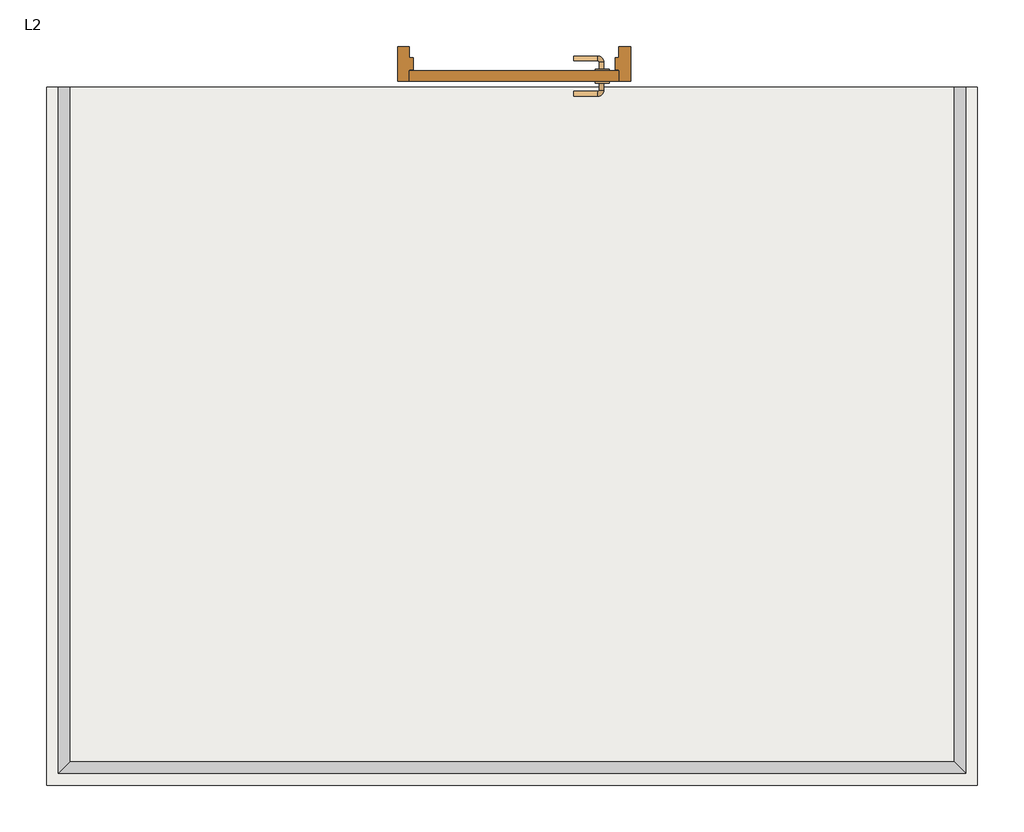
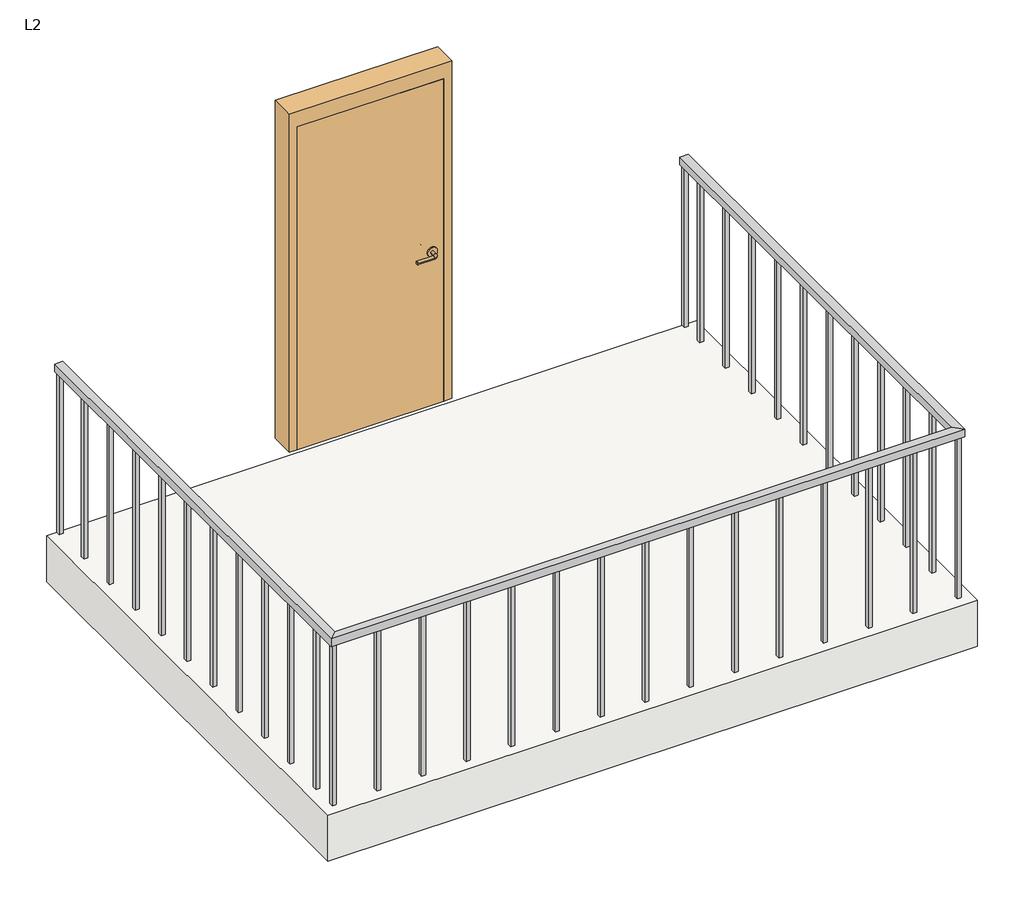
# One storey: 1 door, 1 railing, 1 slab.
"""IFC4 building model written with IfcOpenShell, lengths in millimetres."""

import ifcopenshell
import ifcopenshell.guid

model = None  # the IFC model being written
_history = None  # IfcOwnerHistory: only IFC2X3 demands one
_inside = {}  # id of a spatial element -> (the spatial element, [elements in it])
_under = {}  # id of a project, library or spatial element -> (it, [spatial elements below it])
_declared = {}  # id of a project -> (the project, [libraries it declares])
_typed = {}  # id of a type object -> (the type object, [elements of that type])
_made_of = {}  # id of a material, layer set ... -> (it, [elements and type objects made of it])


def new_model(schema):
    """Start an empty IFC model of exactly this schema.

    Asked for "IFC4X3", IfcOpenShell would pick the latest addendum, in which some entities
    have other attributes; the version numbers below select the first issue.
    IFC2X3 requires an IfcOwnerHistory on every rooted entity: one is made here for all.
    """
    global model, _history
    if schema == "IFC4X3":
        model = ifcopenshell.file(schema_version=(4, 3, 0, 0))
    else:
        model = ifcopenshell.file(schema=schema)
    _inside.clear()
    _under.clear()
    _declared.clear()
    _typed.clear()
    _made_of.clear()
    _history = None
    if model.schema == "IFC2X3":
        org = make("IfcOrganization", Name="unknown")
        user = make(
            "IfcPersonAndOrganization",
            ThePerson=make("IfcPerson", FamilyName="unknown"),
            TheOrganization=org,
        )
        app = make(
            "IfcApplication",
            ApplicationDeveloper=org,
            Version="unknown",
            ApplicationFullName="unknown",
            ApplicationIdentifier="unknown",
        )
        _history = make(
            "IfcOwnerHistory",
            OwningUser=user,
            OwningApplication=app,
            ChangeAction="ADDED",
            CreationDate=0,
        )
    return model


def make(cls, **values):
    """One entity of the class cls with the attributes given. An attribute that is None is left unset."""
    return model.create_entity(
        cls, **{name: value for name, value in values.items() if value is not None}
    )


def rooted(cls, **values):
    """An entity with a GlobalId (a new one), such as an element, a storey or a relation."""
    return make(cls, GlobalId=ifcopenshell.guid.new(), OwnerHistory=_history, **values)


def si_unit(unit_type, name, prefix=None):
    """IfcSIUnit, for example si_unit("LENGTHUNIT", "METRE", prefix="MILLI")."""
    return make("IfcSIUnit", UnitType=unit_type, Prefix=prefix, Name=name)


def assignment(units):
    """IfcUnitAssignment: the units of a project."""
    return None if units is None else make("IfcUnitAssignment", Units=units)


def point(xyz):
    """IfcCartesianPoint."""
    return None if xyz is None else make("IfcCartesianPoint", Coordinates=xyz)


def direction(xyz):
    """IfcDirection."""
    return None if xyz is None else make("IfcDirection", DirectionRatios=xyz)


def frame(location, z_axis=None, x_axis=None):
    """IfcAxis2Placement3D, a coordinate frame: its origin and axes. An axis left out is left unset."""
    return make(
        "IfcAxis2Placement3D",
        Location=point(location),
        Axis=direction(z_axis),
        RefDirection=direction(x_axis),
    )


def frame_2d(location, x_axis=None):
    """IfcAxis2Placement2D, a coordinate frame in the plane: its origin and x axis."""
    return make(
        "IfcAxis2Placement2D", Location=point(location), RefDirection=direction(x_axis)
    )


def origin():
    """The frame at (0, 0, 0) with its axes left unset."""
    return frame((0.0, 0.0, 0.0))


def origin_with_axes():
    """The frame at (0, 0, 0) with the z axis (0, 0, 1) and the x axis (1, 0, 0) written out."""
    return frame((0.0, 0.0, 0.0), z_axis=(0.0, 0.0, 1.0), x_axis=(1.0, 0.0, 0.0))


def place(relative_to, where):
    """IfcLocalPlacement: puts the frame where relative to a parent placement (None: the world)."""
    return make(
        "IfcLocalPlacement", PlacementRelTo=relative_to, RelativePlacement=where
    )


def context(
    kind, dimensions, precision=None, world=None, true_north=None, identifier=None
):
    """IfcGeometricRepresentationContext, for example the 3D "Model" context."""
    return make(
        "IfcGeometricRepresentationContext",
        ContextIdentifier=identifier,
        ContextType=kind,
        CoordinateSpaceDimension=dimensions,
        Precision=precision,
        WorldCoordinateSystem=world,
        TrueNorth=true_north,
    )


def project(units=None, contexts=None):
    """IfcProject with its units and contexts."""
    return rooted(
        "IfcProject",
        Name="project",
        RepresentationContexts=contexts,
        UnitsInContext=assignment(units),
    )


def spatial(cls, under=None, at=None, **own):
    """A site, building, storey or space (cls), placed at a placement, below another one or the project."""
    s = rooted(cls, ObjectPlacement=at, **own)
    if under is not None:
        _under.setdefault(under.id(), (under, []))[1].append(s)
    return s


def polyline(points):
    """IfcPolyline through the points."""
    return make("IfcPolyline", Points=[point(p) for p in points])


def circle_curve(where, radius):
    """IfcCircle in the frame where."""
    return make("IfcCircle", Position=where, Radius=radius)


def ellipse_curve(where, semi_axis1, semi_axis2):
    """IfcEllipse in the frame where."""
    return make(
        "IfcEllipse", Position=where, SemiAxis1=semi_axis1, SemiAxis2=semi_axis2
    )


def trimmed(basis, trim1, trim2, sense, master):
    """IfcTrimmedCurve: the piece of a basis curve between two trims."""
    return make(
        "IfcTrimmedCurve",
        BasisCurve=basis,
        Trim1=trim1,
        Trim2=trim2,
        SenseAgreement=sense,
        MasterRepresentation=master,
    )


def segment(curve, same_sense, transition):
    """IfcCompositeCurveSegment."""
    return make(
        "IfcCompositeCurveSegment",
        Transition=transition,
        SameSense=same_sense,
        ParentCurve=curve,
    )


def composite_curve(segments, self_intersect=None):
    """IfcCompositeCurve: segments joined end to end."""
    return make("IfcCompositeCurve", Segments=segments, SelfIntersect=self_intersect)


def outline(outer, holes=None, kind="AREA"):
    """IfcArbitraryClosedProfileDef: a profile drawn as a closed curve; with holes, ...WithVoids."""
    if holes is None:
        return make("IfcArbitraryClosedProfileDef", ProfileType=kind, OuterCurve=outer)
    return make(
        "IfcArbitraryProfileDefWithVoids",
        ProfileType=kind,
        OuterCurve=outer,
        InnerCurves=holes,
    )


def extrude(swept, where, along, depth):
    """IfcExtrudedAreaSolid: the profile swept, set in the frame where, extruded along a direction by depth."""
    return make(
        "IfcExtrudedAreaSolid",
        SweptArea=swept,
        Position=where,
        ExtrudedDirection=direction(along),
        Depth=depth,
    )


def faces_of(points, faces, orient=None, outer=None):
    """IfcFace entities. A face is a list of loops; a loop is a list of indices into points, from 0.

    orient and outer hold one flag for each loop. By default every Orientation is true, the
    first loop of a face is its IfcFaceOuterBound and the others are IfcFaceBound.
    """
    made = []
    for i, loops in enumerate(faces):
        bounds = []
        for j, loop in enumerate(loops):
            is_outer = j == 0 if outer is None else outer[i][j]
            bounds.append(
                make(
                    "IfcFaceOuterBound" if is_outer else "IfcFaceBound",
                    Bound=make("IfcPolyLoop", Polygon=[points[k] for k in loop]),
                    Orientation=True if orient is None else orient[i][j],
                )
            )
        made.append(make("IfcFace", Bounds=bounds))
    return made


def faceted_brep(points, faces, orient=None, outer=None, voids=None):
    """IfcFacetedBrep: a solid bounded by flat faces; with voids (closed shells), ...WithVoids."""
    shared = [point(p) for p in points]
    hull = make("IfcClosedShell", CfsFaces=faces_of(shared, faces, orient, outer))
    if voids is None:
        return make("IfcFacetedBrep", Outer=hull)
    return make(
        "IfcFacetedBrepWithVoids",
        Outer=hull,
        Voids=[
            make(cls, CfsFaces=faces_of(shared, fs, o, b)) for cls, fs, o, b in voids
        ],
    )


def shape(context_of_items, identifier, shape_type, items):
    """IfcShapeRepresentation: the items that make up one representation, for example the "Body"."""
    return make(
        "IfcShapeRepresentation",
        ContextOfItems=context_of_items,
        RepresentationIdentifier=identifier,
        RepresentationType=shape_type,
        Items=items,
    )


def source(mapping_origin, context_of_items, identifier, shape_type, items):
    """IfcRepresentationMap: a shape defined once, which mapped items show again and again."""
    return make(
        "IfcRepresentationMap",
        MappingOrigin=mapping_origin,
        MappedRepresentation=shape(context_of_items, identifier, shape_type, items),
    )


def transform(
    local_origin,
    x_axis=None,
    y_axis=None,
    z_axis=None,
    scale=None,
    scale2=None,
    scale3=None,
    uniform=True,
):
    """IfcCartesianTransformationOperator3D, or its non-uniform kind. x_axis, y_axis, z_axis: its Axis1, 2, 3."""
    if uniform:
        return make(
            "IfcCartesianTransformationOperator3D",
            Axis1=direction(x_axis),
            Axis2=direction(y_axis),
            LocalOrigin=point(local_origin),
            Scale=scale,
            Axis3=direction(z_axis),
        )
    return make(
        "IfcCartesianTransformationOperator3DnonUniform",
        Axis1=direction(x_axis),
        Axis2=direction(y_axis),
        LocalOrigin=point(local_origin),
        Scale=scale,
        Axis3=direction(z_axis),
        Scale2=scale2,
        Scale3=scale3,
    )


def mapped(mapping_source, mapping_target):
    """IfcMappedItem: shows the shape of a source again, moved by a transform."""
    return make(
        "IfcMappedItem", MappingSource=mapping_source, MappingTarget=mapping_target
    )


def made_of(thing, what):
    """Note that an element or type object is made of a material, layer set ...; save() writes the relation."""
    if what is not None:
        _made_of.setdefault(what.id(), (what, []))[1].append(thing)
    return thing


def element(
    cls,
    number,
    at=None,
    inside=None,
    cuts=None,
    type_object=None,
    material=None,
    context=None,
    identifier="Body",
    shape_type=None,
    held_by="IfcProductDefinitionShape",
    body=None,
    shapes=None,
    **own,
):
    """One element of the class cls, such as IfcWall. Its Tag is "e" and its number.

    at: its placement. inside: the storey or other place that contains it. cuts: it is an
    opening in that element (IfcRelVoidsElement). A single representation is given by context,
    identifier, shape_type and body (its items); several are given by shapes. held_by: the class
    of the entity that holds the representations. save() writes the other relations.
    """
    e = rooted(cls, Tag="e%d" % number, ObjectPlacement=at, **own)
    if body is not None:
        shapes = [shape(context, identifier, shape_type, body)]
    if shapes is not None:
        e.Representation = make(held_by, Representations=shapes)
    if inside is not None:
        _inside.setdefault(inside.id(), (inside, []))[1].append(e)
    if cuts is not None:
        rooted(
            "IfcRelVoidsElement", RelatingBuildingElement=cuts, RelatedOpeningElement=e
        )
    if type_object is not None:
        _typed.setdefault(type_object.id(), (type_object, []))[1].append(e)
    return made_of(e, material)


def aggregate(whole, parts):
    """IfcRelAggregates: a whole, such as a stair, and the parts it consists of."""
    return rooted("IfcRelAggregates", RelatingObject=whole, RelatedObjects=parts)


def save(model, path):
    """Write the relations noted so far, then the file.

    IfcRelAggregates (storeys below a building ...), IfcRelContainedInSpatialStructure (elements
    in a storey), IfcRelDefinesByType, IfcRelAssociatesMaterial and IfcRelDeclares: one each for
    every whole, place, type object, material and project.
    """
    for whole, parts in _under.values():
        aggregate(whole, parts)
    for where, things in _inside.values():
        rooted(
            "IfcRelContainedInSpatialStructure",
            RelatedElements=things,
            RelatingStructure=where,
        )
    for kind, things in _typed.values():
        rooted("IfcRelDefinesByType", RelatedObjects=things, RelatingType=kind)
    for what, things in _made_of.values():
        rooted("IfcRelAssociatesMaterial", RelatedObjects=things, RelatingMaterial=what)
    for by, libraries in _declared.values():
        rooted("IfcRelDeclares", RelatingContext=by, RelatedDefinitions=libraries)
    model.write(path)


def plane_surface(at):
    """IfcPlane: the flat surface through the origin of the frame at, square to its z axis."""
    return make("IfcPlane", Position=at)


def cylinder_surface(at, radius):
    """IfcCylindricalSurface: all points at the distance radius from the z axis of the frame at."""
    return make("IfcCylindricalSurface", Position=at, Radius=radius)


def revolved_surface(curve, axis_point, axis_direction):
    """IfcSurfaceOfRevolution: the curve turned about the line through axis_point along axis_direction."""
    return make(
        "IfcSurfaceOfRevolution",
        SweptCurve=make("IfcArbitraryOpenProfileDef", ProfileType="CURVE", Curve=curve),
        AxisPosition=make("IfcAxis1Placement", Location=point(axis_point), Axis=direction(axis_direction)),
    )


def advanced_brep(points, edges, surfaces, faces):
    """IfcAdvancedBrep: a solid bounded by faces that lie on surfaces and meet in shared edges.

    An edge is (start, end): straight between two places in points (the first is 0);
    or (start, end, curve); or (start, end, curve, False) where it runs against its curve.
    A face is (place in surfaces, loops), or (place, loops, False) where it looks against
    its surface's normal. A loop lists edges by number (the first is 1), with a minus sign
    where the edge is run from its end to its start. The first loop is the outer one.
    """
    corners = [point(p) for p in points]
    vertices = [make("IfcVertexPoint", VertexGeometry=c) for c in corners]
    made = []
    for start, end, *more in edges:
        made.append(
            make(
                "IfcEdgeCurve",
                EdgeStart=vertices[start],
                EdgeEnd=vertices[end],
                EdgeGeometry=more[0] if more else make("IfcPolyline", Points=[corners[start], corners[end]]),
                SameSense=more[1] if len(more) > 1 else True,
            )
        )
    hull = []
    for where, loops, *sense in faces:
        bounds = []
        for j, loop in enumerate(loops):
            ring = [make("IfcOrientedEdge", EdgeElement=made[abs(k) - 1], Orientation=k > 0) for k in loop]
            bounds.append(
                make(
                    "IfcFaceOuterBound" if j == 0 else "IfcFaceBound",
                    Bound=make("IfcEdgeLoop", EdgeList=ring),
                    Orientation=True,
                )
            )
        hull.append(make("IfcAdvancedFace", Bounds=bounds, FaceSurface=surfaces[where], SameSense=sense[0] if sense else True))
    return make("IfcAdvancedBrep", Outer=make("IfcClosedShell", CfsFaces=hull))


def m_door_passage_single_flush_900_x_2100mm_f70d95c9(model_context):
    return source(origin(), model_context, "Body", "SolidModel", [
        advanced_brep(
        [(-384.990625, 3.35, 1000.0), (-364.990625, 3.35, 1000.0), (-364.990625, -26.65, 1000.0), (-384.990625, -26.65, 1000.0), (-359.990625, -31.65, 1000.0), (-359.990625, -51.65, 1000.0), (-254.990625, -51.65, 1000.0), (-254.990625, -31.65, 1000.0)],
        [
            (0, 1, circle_curve(frame((-374.990625, 3.35, 1000.0), z_axis=(0.0, 1.0, 0.0), x_axis=(1.0, 0.0, 0.0)), 10.0)),
            (1, 0, circle_curve(frame((-374.990625, 3.35, 1000.0), z_axis=(0.0, 1.0, 0.0), x_axis=(1.0, 0.0, 0.0)), 10.0)),
            (1, 2),
            (2, 3, circle_curve(frame((-374.990625, -26.65, 1000.0), z_axis=(0.0, 1.0, 0.0), x_axis=(1.0, 0.0, 0.0)), 10.0)),
            (3, 0),
            (3, 2, circle_curve(frame((-374.990625, -26.65, 1000.0), z_axis=(0.0, 1.0, 0.0), x_axis=(1.0, 0.0, 0.0)), 10.0)),
            (4, 5, circle_curve(frame((-359.990625, -41.65, 1000.0), z_axis=(-1.0, 0.0, 0.0), x_axis=(0.0, 1.0, 0.0)), 10.0)),
            (5, 3, circle_curve(frame((-359.990625, -26.65, 1000.0), z_axis=(0.0, 0.0, -1.0), x_axis=(-1.0, 0.0, 0.0)), 25.0)),
            (2, 4, circle_curve(frame((-359.990625, -26.65, 1000.0), z_axis=(0.0, 0.0, 1.0), x_axis=(-1.0, 0.0, 0.0)), 5.0)),
            (5, 4, circle_curve(frame((-359.990625, -41.65, 1000.0), z_axis=(-1.0, 0.0, 0.0), x_axis=(0.0, 1.0, 0.0)), 10.0)),
            (6, 7, circle_curve(frame((-254.990625, -41.65, 1000.0), z_axis=(1.0, 0.0, 0.0), x_axis=(0.0, 1.0, 0.0)), 10.0)),
            (7, 6, circle_curve(frame((-254.990625, -41.65, 1000.0), z_axis=(1.0, 0.0, 0.0), x_axis=(0.0, 1.0, 0.0)), 10.0)),
            (4, 7),
            (6, 5),
        ],
        [
            plane_surface(frame((-374.990625, 3.35, 1000.0), z_axis=(0.0, 1.0, 0.0), x_axis=(0.0, 0.0, 1.0))),
            cylinder_surface(frame((-374.990625, 3.35, 1000.0), z_axis=(0.0, 1.0, 0.0), x_axis=(1.0, 0.0, 0.0)), 10.0),
            revolved_surface(trimmed(ellipse_curve(frame((-374.990625, -26.65, 1000.0), z_axis=(0.0, -1.0, 0.0), x_axis=(1.0, 0.0, 0.0)), 10.0, 10.0), [point((-384.990625, -26.65, 1000.0))], [point((-364.990625, -26.65, 1000.0))], True, "CARTESIAN"), (-359.990625, -26.65, 1000.0), (0.0, 0.0, -1.0)),
            revolved_surface(trimmed(ellipse_curve(frame((-374.990625, -26.65, 1000.0), z_axis=(0.0, -1.0, 0.0), x_axis=(1.0, 0.0, 0.0)), 10.0, 10.0), [point((-364.990625, -26.65, 1000.0))], [point((-384.990625, -26.65, 1000.0))], True, "CARTESIAN"), (-359.990625, -26.65, 1000.0), (0.0, 0.0, -1.0)),
            plane_surface(frame((-254.990625, -41.65, 1000.0), z_axis=(1.0, 0.0, 0.0), x_axis=(0.0, 0.0, 1.0))),
            cylinder_surface(frame((-359.990625, -41.65, 1000.0), z_axis=(-1.0, 0.0, 0.0), x_axis=(0.0, 1.0, 0.0)), 10.0),
        ],
        [
            (0, [[1, 2]]),
            (1, [[3, 4, 5, -2]]),
            (1, [[-5, 6, -3, -1]]),
            (2, [[7, 8, -4, 9]]),
            (3, [[10, -9, -6, -8]]),
            (4, [[11, 12]]),
            (5, [[13, -11, 14, -7]]),
            (5, [[-14, -12, -13, -10]]),
        ],
    ),
        extrude(outline(composite_curve([segment(trimmed(circle_curve(frame_2d((1000.0, -377.490625)), 30.0), [point((1000.0, -407.490625))], [point((1000.0, -347.490625))], False, "CARTESIAN"), True, "CONTINUOUS"), segment(trimmed(circle_curve(frame_2d((1000.0, -377.490625)), 30.0), [point((1000.0, -347.490625))], [point((1000.0, -407.490625))], False, "CARTESIAN"), True, "CONTINUOUS")], self_intersect=False)), frame((0.0, 3.35, 0.0), z_axis=(0.0, 1.0, 0.0), x_axis=(0.0, 0.0, 1.0)), (0.0, 0.0, 1.0), 8.0),
        advanced_brep(
        [(-384.990625, 64.35, 1000.0), (-364.990625, 64.35, 1000.0), (-384.990625, 94.35, 1000.0), (-364.990625, 94.35, 1000.0), (-359.990625, 99.35, 1000.0), (-359.990625, 119.35, 1000.0), (-254.990625, 119.35, 1000.0), (-254.990625, 99.35, 1000.0)],
        [
            (0, 1, circle_curve(frame((-374.990625, 64.35, 1000.0), z_axis=(0.0, -1.0, 0.0), x_axis=(1.0, 0.0, 0.0)), 10.0)),
            (1, 0, circle_curve(frame((-374.990625, 64.35, 1000.0), z_axis=(0.0, -1.0, 0.0), x_axis=(1.0, 0.0, 0.0)), 10.0)),
            (0, 2),
            (2, 3, circle_curve(frame((-374.990625, 94.35, 1000.0), z_axis=(0.0, -1.0, 0.0), x_axis=(1.0, 0.0, 0.0)), 10.0)),
            (3, 1),
            (3, 2, circle_curve(frame((-374.990625, 94.35, 1000.0), z_axis=(0.0, -1.0, 0.0), x_axis=(1.0, 0.0, 0.0)), 10.0)),
            (4, 3, circle_curve(frame((-359.990625, 94.35, 1000.0), z_axis=(0.0, 0.0, 1.0), x_axis=(-1.0, 0.0, 0.0)), 5.0)),
            (2, 5, circle_curve(frame((-359.990625, 94.35, 1000.0), z_axis=(0.0, 0.0, -1.0), x_axis=(-1.0, 0.0, 0.0)), 25.0)),
            (5, 4, circle_curve(frame((-359.990625, 109.35, 1000.0), z_axis=(-1.0, 0.0, 0.0), x_axis=(0.0, -1.0, 0.0)), 10.0)),
            (4, 5, circle_curve(frame((-359.990625, 109.35, 1000.0), z_axis=(-1.0, 0.0, 0.0), x_axis=(0.0, -1.0, 0.0)), 10.0)),
            (6, 7, circle_curve(frame((-254.990625, 109.35, 1000.0), z_axis=(1.0, 0.0, 0.0), x_axis=(0.0, -1.0, 0.0)), 10.0)),
            (7, 6, circle_curve(frame((-254.990625, 109.35, 1000.0), z_axis=(1.0, 0.0, 0.0), x_axis=(0.0, -1.0, 0.0)), 10.0)),
            (5, 6),
            (7, 4),
        ],
        [
            plane_surface(frame((-374.990625, 64.35, 1000.0), z_axis=(0.0, -1.0, 0.0), x_axis=(0.0, 0.0, 1.0))),
            cylinder_surface(frame((-374.990625, 64.35, 1000.0), z_axis=(0.0, -1.0, 0.0), x_axis=(1.0, 0.0, 0.0)), 10.0),
            revolved_surface(trimmed(ellipse_curve(frame((-374.990625, 94.35, 1000.0), z_axis=(0.0, -1.0, 0.0), x_axis=(1.0, 0.0, 0.0)), 10.0, 10.0), [point((-384.990625, 94.35, 1000.0))], [point((-364.990625, 94.35, 1000.0))], True, "CARTESIAN"), (-359.990625, 94.35, 1000.0), (0.0, 0.0, -1.0)),
            revolved_surface(trimmed(ellipse_curve(frame((-374.990625, 94.35, 1000.0), z_axis=(0.0, -1.0, 0.0), x_axis=(1.0, 0.0, 0.0)), 10.0, 10.0), [point((-364.990625, 94.35, 1000.0))], [point((-384.990625, 94.35, 1000.0))], True, "CARTESIAN"), (-359.990625, 94.35, 1000.0), (0.0, 0.0, -1.0)),
            plane_surface(frame((-254.990625, 109.35, 1000.0), z_axis=(1.0, 0.0, 0.0), x_axis=(0.0, 0.0, 1.0))),
            cylinder_surface(frame((-359.990625, 109.35, 1000.0), z_axis=(-1.0, 0.0, 0.0), x_axis=(0.0, -1.0, 0.0)), 10.0),
        ],
        [
            (0, [[1, 2]]),
            (1, [[-1, 3, 4, 5]]),
            (1, [[-2, -5, 6, -3]]),
            (2, [[7, -4, 8, 9]]),
            (3, [[-8, -6, -7, 10]]),
            (4, [[11, 12]]),
            (5, [[-9, 13, -12, 14]]),
            (5, [[-10, -14, -11, -13]]),
        ],
    ),
        extrude(outline(composite_curve([segment(trimmed(circle_curve(frame_2d((1000.0, -377.490625)), 30.0), [point((1000.0, -407.490625))], [point((1000.0, -347.490625))], False, "CARTESIAN"), True, "CONTINUOUS"), segment(trimmed(circle_curve(frame_2d((1000.0, -377.490625)), 30.0), [point((1000.0, -347.490625))], [point((1000.0, -407.490625))], False, "CARTESIAN"), True, "CONTINUOUS")], self_intersect=False)), frame((0.0, 56.35, 0.0), z_axis=(0.0, 1.0, 0.0), x_axis=(0.0, 0.0, 1.0)), (0.0, 0.0, 1.0), 8.0),
        extrude(outline(polyline([(450.0, 11.35), (-450.0, 11.35), (-450.0, 56.35), (450.0, 56.35), (450.0, 11.35)])), origin_with_axes(), (0.0, 0.0, 1.0), 2100.0),
        faceted_brep([(450.0, 6.5875, 0.0), (450.0, 56.35, 0.0), (500.0, 56.35, 0.0), (500.0, -93.65, 0.0), (450.0, -93.65, 0.0), (450.0, -44.4375, 0.0), (434.125, -44.4375, 0.0), (434.125, 6.5875, 0.0), (450.0, 6.5875, 2100.0), (450.0, 56.35, 2100.0), (-450.0, 56.35, 2100.0), (-450.0, 56.35, 0.0), (-500.0, 56.35, 0.0), (-500.0, 56.35, 2200.0), (500.0, 56.35, 2200.0), (500.0, -93.65, 2200.0), (-500.0, -93.65, 2200.0), (-500.0, -93.65, 0.0), (-450.0, -93.65, 0.0), (-450.0, -93.65, 2100.0), (450.0, -93.65, 2100.0), (450.0, -44.4375, 2100.0), (-450.0, -44.4375, 2100.0), (-450.0, -44.4375, 0.0), (-434.125, -44.4375, 0.0), (-434.125, -44.4375, 2084.125), (434.125, -44.4375, 2084.125), (434.125, 6.5875, 2084.125), (-434.125, 6.5875, 2084.125), (-434.125, 6.5875, 0.0), (-450.0, 6.5875, 0.0), (-450.0, 6.5875, 2100.0)], [[[0, 1, 2, 3, 4, 5, 6, 7]], [[1, 0, 8, 9]], [[2, 1, 9, 10, 11, 12, 13, 14]], [[3, 2, 14, 15]], [[4, 3, 15, 16, 17, 18, 19, 20]], [[5, 4, 20, 21]], [[6, 5, 21, 22, 23, 24, 25, 26]], [[7, 6, 26, 27]], [[0, 7, 27, 28, 29, 30, 31, 8]], [[9, 8, 31, 10]], [[20, 19, 22, 21]], [[26, 25, 28, 27]], [[12, 11, 30, 29, 24, 23, 18, 17]], [[11, 10, 31, 30]], [[13, 12, 17, 16]], [[19, 18, 23, 22]], [[25, 24, 29, 28]], [[15, 14, 13, 16]]]),
    ])


model = new_model("IFC4")

# Units and contexts
model_context = context("Model", 3, world=origin())
ifc_project = project(units=[si_unit("LENGTHUNIT", "METRE", prefix="MILLI")], contexts=[model_context])

# Site, building, storey
site = spatial("IfcSite", under=ifc_project)
building = spatial("IfcBuilding", under=site)
storey = spatial("IfcBuildingStorey", under=building, Name="L2", Elevation=1200.0)

# Door
placement = place(None, origin())
m_door_passage_single_flush_900_x_2100mm_shape = m_door_passage_single_flush_900_x_2100mm_f70d95c9(model_context)
element("IfcDoor", 1, ObjectType="M_Door-Passage-Single-Flush : 900 x 2100mm", at=placement, inside=storey, context=model_context, shape_type="MappedRepresentation", body=[
    mapped(m_door_passage_single_flush_900_x_2100mm_shape, transform((752.7568, 2222.9207088, 1200.0), x_axis=(-1.0, 0.0, 0.0), y_axis=(0.0, -1.0, 0.0), z_axis=(0.0, 0.0, 1.0))),
])

# Railing
element("IfcRailing", 2, ObjectType="1100mm", at=placement, inside=storey, context=model_context, shape_type="SolidModel", body=[
    faceted_brep([(-1156.7682, 2141.5707088, 2300.0), (-1156.7682, 2141.5707088, 2250.0), (-1206.7682, 2141.5707088, 2250.0), (-1206.7682, 2141.5707088, 2300.0), (-1156.7682, -758.4292912, 2300.0), (-1156.7682, -758.4292912, 2250.0), (-1206.7682, -808.4292912, 2250.0), (-1206.7682, -808.4292912, 2300.0), (2643.2318, -758.4292912, 2300.0), (2643.2318, -758.4292912, 2250.0), (2693.2318, -808.4292912, 2250.0), (2693.2318, -808.4292912, 2300.0), (2643.2318, 2141.5707088, 2300.0), (2693.2318, 2141.5707088, 2300.0), (2693.2318, 2141.5707088, 2250.0), (2643.2318, 2141.5707088, 2250.0)], [[[0, 1, 2, 3]], [[1, 0, 4, 5]], [[2, 1, 5, 6]], [[3, 2, 6, 7]], [[0, 3, 7, 4]], [[5, 4, 8, 9]], [[6, 5, 9, 10]], [[7, 6, 10, 11]], [[4, 7, 11, 8]], [[12, 13, 14, 15]], [[9, 8, 12, 15]], [[10, 9, 15, 14]], [[11, 10, 14, 13]], [[8, 11, 13, 12]]]),
    extrude(outline(polyline([(2680.7318, 1954.0707088), (2655.7318, 1954.0707088), (2655.7318, 1979.0707088), (2680.7318, 1979.0707088), (2680.7318, 1954.0707088)])), frame((0.0, 0.0, 1200.0), z_axis=(0.0, 0.0, 1.0), x_axis=(1.0, 0.0, 0.0)), (0.0, 0.0, 1.0), 1050.0),
    extrude(outline(polyline([(2680.7318, 1679.0707088), (2655.7318, 1679.0707088), (2655.7318, 1704.0707088), (2680.7318, 1704.0707088), (2680.7318, 1679.0707088)])), frame((0.0, 0.0, 1200.0), z_axis=(0.0, 0.0, 1.0), x_axis=(1.0, 0.0, 0.0)), (0.0, 0.0, 1.0), 1050.0),
    extrude(outline(polyline([(2680.7318, 1404.0707088), (2655.7318, 1404.0707088), (2655.7318, 1429.0707088), (2680.7318, 1429.0707088), (2680.7318, 1404.0707088)])), frame((0.0, 0.0, 1200.0), z_axis=(0.0, 0.0, 1.0), x_axis=(1.0, 0.0, 0.0)), (0.0, 0.0, 1.0), 1050.0),
    extrude(outline(polyline([(2680.7318, 1129.0707088), (2655.7318, 1129.0707088), (2655.7318, 1154.0707088), (2680.7318, 1154.0707088), (2680.7318, 1129.0707088)])), frame((0.0, 0.0, 1200.0), z_axis=(0.0, 0.0, 1.0), x_axis=(1.0, 0.0, 0.0)), (0.0, 0.0, 1.0), 1050.0),
    extrude(outline(polyline([(2680.7318, 854.0707088), (2655.7318, 854.0707088), (2655.7318, 879.0707088), (2680.7318, 879.0707088), (2680.7318, 854.0707088)])), frame((0.0, 0.0, 1200.0), z_axis=(0.0, 0.0, 1.0), x_axis=(1.0, 0.0, 0.0)), (0.0, 0.0, 1.0), 1050.0),
    extrude(outline(polyline([(2680.7318, 579.0707088), (2655.7318, 579.0707088), (2655.7318, 604.0707088), (2680.7318, 604.0707088), (2680.7318, 579.0707088)])), frame((0.0, 0.0, 1200.0), z_axis=(0.0, 0.0, 1.0), x_axis=(1.0, 0.0, 0.0)), (0.0, 0.0, 1.0), 1050.0),
    extrude(outline(polyline([(2680.7318, 304.0707088), (2655.7318, 304.0707088), (2655.7318, 329.0707088), (2680.7318, 329.0707088), (2680.7318, 304.0707088)])), frame((0.0, 0.0, 1200.0), z_axis=(0.0, 0.0, 1.0), x_axis=(1.0, 0.0, 0.0)), (0.0, 0.0, 1.0), 1050.0),
    extrude(outline(polyline([(2680.7318, 29.0707088), (2655.7318, 29.0707088), (2655.7318, 54.0707088), (2680.7318, 54.0707088), (2680.7318, 29.0707088)])), frame((0.0, 0.0, 1200.0), z_axis=(0.0, 0.0, 1.0), x_axis=(1.0, 0.0, 0.0)), (0.0, 0.0, 1.0), 1050.0),
    extrude(outline(polyline([(2680.7318, -245.9292912), (2655.7318, -245.9292912), (2655.7318, -220.9292912), (2680.7318, -220.9292912), (2680.7318, -245.9292912)])), frame((0.0, 0.0, 1200.0), z_axis=(0.0, 0.0, 1.0), x_axis=(1.0, 0.0, 0.0)), (0.0, 0.0, 1.0), 1050.0),
    extrude(outline(polyline([(2680.7318, -520.9292912), (2655.7318, -520.9292912), (2655.7318, -495.9292912), (2680.7318, -495.9292912), (2680.7318, -520.9292912)])), frame((0.0, 0.0, 1200.0), z_axis=(0.0, 0.0, 1.0), x_axis=(1.0, 0.0, 0.0)), (0.0, 0.0, 1.0), 1050.0),
    extrude(outline(polyline([(2380.7318, -795.9292912), (2380.7318, -770.9292912), (2405.7318, -770.9292912), (2405.7318, -795.9292912), (2380.7318, -795.9292912)])), frame((0.0, 0.0, 1200.0), z_axis=(0.0, 0.0, 1.0), x_axis=(1.0, 0.0, 0.0)), (0.0, 0.0, 1.0), 1050.0),
    extrude(outline(polyline([(2105.7318, -795.9292912), (2105.7318, -770.9292912), (2130.7318, -770.9292912), (2130.7318, -795.9292912), (2105.7318, -795.9292912)])), frame((0.0, 0.0, 1200.0), z_axis=(0.0, 0.0, 1.0), x_axis=(1.0, 0.0, 0.0)), (0.0, 0.0, 1.0), 1050.0),
    extrude(outline(polyline([(1830.7318, -795.9292912), (1830.7318, -770.9292912), (1855.7318, -770.9292912), (1855.7318, -795.9292912), (1830.7318, -795.9292912)])), frame((0.0, 0.0, 1200.0), z_axis=(0.0, 0.0, 1.0), x_axis=(1.0, 0.0, 0.0)), (0.0, 0.0, 1.0), 1050.0),
    extrude(outline(polyline([(1555.7318, -795.9292912), (1555.7318, -770.9292912), (1580.7318, -770.9292912), (1580.7318, -795.9292912), (1555.7318, -795.9292912)])), frame((0.0, 0.0, 1200.0), z_axis=(0.0, 0.0, 1.0), x_axis=(1.0, 0.0, 0.0)), (0.0, 0.0, 1.0), 1050.0),
    extrude(outline(polyline([(1280.7318, -795.9292912), (1280.7318, -770.9292912), (1305.7318, -770.9292912), (1305.7318, -795.9292912), (1280.7318, -795.9292912)])), frame((0.0, 0.0, 1200.0), z_axis=(0.0, 0.0, 1.0), x_axis=(1.0, 0.0, 0.0)), (0.0, 0.0, 1.0), 1050.0),
    extrude(outline(polyline([(1005.7318, -795.9292912), (1005.7318, -770.9292912), (1030.7318, -770.9292912), (1030.7318, -795.9292912), (1005.7318, -795.9292912)])), frame((0.0, 0.0, 1200.0), z_axis=(0.0, 0.0, 1.0), x_axis=(1.0, 0.0, 0.0)), (0.0, 0.0, 1.0), 1050.0),
    extrude(outline(polyline([(730.7318, -795.9292912), (730.7318, -770.9292912), (755.7318, -770.9292912), (755.7318, -795.9292912), (730.7318, -795.9292912)])), frame((0.0, 0.0, 1200.0), z_axis=(0.0, 0.0, 1.0), x_axis=(1.0, 0.0, 0.0)), (0.0, 0.0, 1.0), 1050.0),
    extrude(outline(polyline([(455.7318, -795.9292912), (455.7318, -770.9292912), (480.7318, -770.9292912), (480.7318, -795.9292912), (455.7318, -795.9292912)])), frame((0.0, 0.0, 1200.0), z_axis=(0.0, 0.0, 1.0), x_axis=(1.0, 0.0, 0.0)), (0.0, 0.0, 1.0), 1050.0),
    extrude(outline(polyline([(180.7318, -795.9292912), (180.7318, -770.9292912), (205.7318, -770.9292912), (205.7318, -795.9292912), (180.7318, -795.9292912)])), frame((0.0, 0.0, 1200.0), z_axis=(0.0, 0.0, 1.0), x_axis=(1.0, 0.0, 0.0)), (0.0, 0.0, 1.0), 1050.0),
    extrude(outline(polyline([(-94.2682, -795.9292912), (-94.2682, -770.9292912), (-69.2682, -770.9292912), (-69.2682, -795.9292912), (-94.2682, -795.9292912)])), frame((0.0, 0.0, 1200.0), z_axis=(0.0, 0.0, 1.0), x_axis=(1.0, 0.0, 0.0)), (0.0, 0.0, 1.0), 1050.0),
    extrude(outline(polyline([(-369.2682, -795.9292912), (-369.2682, -770.9292912), (-344.2682, -770.9292912), (-344.2682, -795.9292912), (-369.2682, -795.9292912)])), frame((0.0, 0.0, 1200.0), z_axis=(0.0, 0.0, 1.0), x_axis=(1.0, 0.0, 0.0)), (0.0, 0.0, 1.0), 1050.0),
    extrude(outline(polyline([(-644.2682, -795.9292912), (-644.2682, -770.9292912), (-619.2682, -770.9292912), (-619.2682, -795.9292912), (-644.2682, -795.9292912)])), frame((0.0, 0.0, 1200.0), z_axis=(0.0, 0.0, 1.0), x_axis=(1.0, 0.0, 0.0)), (0.0, 0.0, 1.0), 1050.0),
    extrude(outline(polyline([(-919.2682, -795.9292912), (-919.2682, -770.9292912), (-894.2682, -770.9292912), (-894.2682, -795.9292912), (-919.2682, -795.9292912)])), frame((0.0, 0.0, 1200.0), z_axis=(0.0, 0.0, 1.0), x_axis=(1.0, 0.0, 0.0)), (0.0, 0.0, 1.0), 1050.0),
    extrude(outline(polyline([(-1194.2682, -595.9292912), (-1169.2682, -595.9292912), (-1169.2682, -620.9292912), (-1194.2682, -620.9292912), (-1194.2682, -595.9292912)])), frame((0.0, 0.0, 1200.0), z_axis=(0.0, 0.0, 1.0), x_axis=(1.0, 0.0, 0.0)), (0.0, 0.0, 1.0), 1050.0),
    extrude(outline(polyline([(-1194.2682, -320.9292912), (-1169.2682, -320.9292912), (-1169.2682, -345.9292912), (-1194.2682, -345.9292912), (-1194.2682, -320.9292912)])), frame((0.0, 0.0, 1200.0), z_axis=(0.0, 0.0, 1.0), x_axis=(1.0, 0.0, 0.0)), (0.0, 0.0, 1.0), 1050.0),
    extrude(outline(polyline([(-1194.2682, -45.9292912), (-1169.2682, -45.9292912), (-1169.2682, -70.9292912), (-1194.2682, -70.9292912), (-1194.2682, -45.9292912)])), frame((0.0, 0.0, 1200.0), z_axis=(0.0, 0.0, 1.0), x_axis=(1.0, 0.0, 0.0)), (0.0, 0.0, 1.0), 1050.0),
    extrude(outline(polyline([(-1194.2682, 229.0707088), (-1169.2682, 229.0707088), (-1169.2682, 204.0707088), (-1194.2682, 204.0707088), (-1194.2682, 229.0707088)])), frame((0.0, 0.0, 1200.0), z_axis=(0.0, 0.0, 1.0), x_axis=(1.0, 0.0, 0.0)), (0.0, 0.0, 1.0), 1050.0),
    extrude(outline(polyline([(-1194.2682, 504.0707088), (-1169.2682, 504.0707088), (-1169.2682, 479.0707088), (-1194.2682, 479.0707088), (-1194.2682, 504.0707088)])), frame((0.0, 0.0, 1200.0), z_axis=(0.0, 0.0, 1.0), x_axis=(1.0, 0.0, 0.0)), (0.0, 0.0, 1.0), 1050.0),
    extrude(outline(polyline([(-1194.2682, 779.0707088), (-1169.2682, 779.0707088), (-1169.2682, 754.0707088), (-1194.2682, 754.0707088), (-1194.2682, 779.0707088)])), frame((0.0, 0.0, 1200.0), z_axis=(0.0, 0.0, 1.0), x_axis=(1.0, 0.0, 0.0)), (0.0, 0.0, 1.0), 1050.0),
    extrude(outline(polyline([(-1194.2682, 1054.0707088), (-1169.2682, 1054.0707088), (-1169.2682, 1029.0707088), (-1194.2682, 1029.0707088), (-1194.2682, 1054.0707088)])), frame((0.0, 0.0, 1200.0), z_axis=(0.0, 0.0, 1.0), x_axis=(1.0, 0.0, 0.0)), (0.0, 0.0, 1.0), 1050.0),
    extrude(outline(polyline([(-1194.2682, 1329.0707088), (-1169.2682, 1329.0707088), (-1169.2682, 1304.0707088), (-1194.2682, 1304.0707088), (-1194.2682, 1329.0707088)])), frame((0.0, 0.0, 1200.0), z_axis=(0.0, 0.0, 1.0), x_axis=(1.0, 0.0, 0.0)), (0.0, 0.0, 1.0), 1050.0),
    extrude(outline(polyline([(-1194.2682, 1604.0707088), (-1169.2682, 1604.0707088), (-1169.2682, 1579.0707088), (-1194.2682, 1579.0707088), (-1194.2682, 1604.0707088)])), frame((0.0, 0.0, 1200.0), z_axis=(0.0, 0.0, 1.0), x_axis=(1.0, 0.0, 0.0)), (0.0, 0.0, 1.0), 1050.0),
    extrude(outline(polyline([(-1194.2682, 1879.0707088), (-1169.2682, 1879.0707088), (-1169.2682, 1854.0707088), (-1194.2682, 1854.0707088), (-1194.2682, 1879.0707088)])), frame((0.0, 0.0, 1200.0), z_axis=(0.0, 0.0, 1.0), x_axis=(1.0, 0.0, 0.0)), (0.0, 0.0, 1.0), 1050.0),
    extrude(outline(polyline([(2655.7318, -795.9292912), (2655.7318, -770.9292912), (2680.7318, -770.9292912), (2680.7318, -795.9292912), (2655.7318, -795.9292912)])), frame((0.0, 0.0, 1200.0), z_axis=(0.0, 0.0, 1.0), x_axis=(1.0, 0.0, 0.0)), (0.0, 0.0, 1.0), 1050.0),
    extrude(outline(polyline([(-1194.2682, -770.9292912), (-1169.2682, -770.9292912), (-1169.2682, -795.9292912), (-1194.2682, -795.9292912), (-1194.2682, -770.9292912)])), frame((0.0, 0.0, 1200.0), z_axis=(0.0, 0.0, 1.0), x_axis=(1.0, 0.0, 0.0)), (0.0, 0.0, 1.0), 1050.0),
    extrude(outline(polyline([(2680.7318, 2116.5707088), (2655.7318, 2116.5707088), (2655.7318, 2141.5707088), (2680.7318, 2141.5707088), (2680.7318, 2116.5707088)])), frame((0.0, 0.0, 1200.0), z_axis=(0.0, 0.0, 1.0), x_axis=(1.0, 0.0, 0.0)), (0.0, 0.0, 1.0), 1050.0),
    extrude(outline(polyline([(-1194.2682, 2141.5707088), (-1169.2682, 2141.5707088), (-1169.2682, 2116.5707088), (-1194.2682, 2116.5707088), (-1194.2682, 2141.5707088)])), frame((0.0, 0.0, 1200.0), z_axis=(0.0, 0.0, 1.0), x_axis=(1.0, 0.0, 0.0)), (0.0, 0.0, 1.0), 1050.0),
])

# Slab
element("IfcSlab", 3, ObjectType="Generic 300mm", at=placement, inside=storey, context=model_context, shape_type="SweptSolid", body=[
    extrude(outline(polyline([(2743.2318, -858.4292912), (-1256.7682, -858.4292912), (-1256.7682, 2141.5707088), (2743.2318, 2141.5707088), (2743.2318, -858.4292912)])), frame((0.0, 0.0, 900.0), z_axis=(0.0, 0.0, 1.0), x_axis=(1.0, 0.0, 0.0)), (0.0, 0.0, 1.0), 300.0),
])

save(model, "model.ifc")

# Revit data of these elements
# Project information
#   Название организации = "Organization Name"
#   Описание организации = "Organization Description"
#   Наименование здания = "Building Name"
#   Дата утверждения проекта = "Issue Date"
#   Статус проекта = "Project Status"
#   Заказчик = "Client Name"
#   Адрес проекта = "Enter address here\nAddress Line 2"
#   Наименование проекта = "Project Name"
#   Номер проекта = "Project Number"
# Type "M_Door-Passage-Single-Flush : 900 x 2100mm"
#   Type Mark = "38"
#   Analytic Construction = "Wooden"
#   Thickness = 45 mm
#   Thermal Resistance (R) = 0.455703 (m²·K)/W
#   Swing Angle [instance default] = 90.00°
#   Strike Height = 1000 mm
#   Rough Width [instance default] = 1000 mm
#   Rough Height [instance default] = 2200 mm
#   MF Opening Height [instance default] = 100 mm
#   MF Opening Width [instance default] = 100 mm
#   Inset Calculate [instance default] = 105 mm
#   Masonry Inset [instance default] = 25 mm
#   Height = 2100 mm
#   Width = 900 mm
#   Heat Transfer Coefficient (U) = 2.19465 W/(m²·K)
#   Masonry Frame Depth = 150 mm
#   Masonry Frame [instance default] = yes
#   Function = 1
#   Dry Wall Frame [instance default] = no
#   Panel Material = Wood - Birch
#   Frame Material = Metal - Paint Finish - Grey
#   Door Handle Material = Aluminum
#   Visual Light Transmittance = 0
#   Solar Heat Gain Coefficient = 0
#   Wall Closure = (empty or 0)
# Type "1100mm"
#   built-in parameter 1008612 = 0.019685 (stored number, unit not read)
#   built-in parameter 1008611 = 0.019685 (stored number, unit not read)
#   built-in parameter 1008609 = 0.902231 (stored number, unit not read)
#   built-in parameter 1008604 = 0.19685 (stored number, unit not read)
#   built-in parameter 1008603 = 0.164042 (stored number, unit not read)
#   Railing Height = 1100 mm
#   built-in parameter 1008630 = 2
#   built-in parameter 1008610 = 2
#   built-in parameter 1008608 = 1
#   built-in parameter 1008618 = M_Baluster - Square : 25mm
# Type "Generic 300mm"
#   Description = "Generic Floor (Material By Category), 300mm thick"
#   Function = 0
#   Layers, outside or top first: 300 mm no material (function 1)
# Element 1 (IfcDoor, "M_Door-Passage-Single-Flush : 900 x 2100mm")
#   Swing Angle = 90.00°
#   Rough Width = 1000 mm
#   Rough Height = 2200 mm
#   Masonry Inset = 25 mm
#   MF Opening Width = 100 mm
#   MF Opening Height = 100 mm
#   Inset Calculate = 105 mm
#   Masonry Frame = yes
#   Dry Wall Frame = no
#   Phase Created = New Construction
#   Materials on its faces: "Aluminum", "Metal - Paint Finish - Grey", "Wood - Birch"
# Element 2 (IfcRailing, "1100mm")
#   Phase Created = New Construction
# Element 3 (IfcSlab, "Generic 300mm")
#   Height Offset From Level = 0 mm
#   Phase Created = New Construction
#   Materials on its faces: "Default Floor"
# Materials
#   "Wood - Birch": class "Wood", colour RGB 173 132 96, transparency 0, Cost = 0
#   "Metal - Paint Finish - Grey": class "Paint", colour RGB 178 178 178, transparency 0, Cost = 0
#   "Aluminum": class "Metal", colour RGB 244 245 246, transparency 0, Description = "Aluminum 6061", Cost = 0
#   "Default Floor": class "Miscellaneous", colour RGB 128 128 128, transparency 0, Cost = 0
